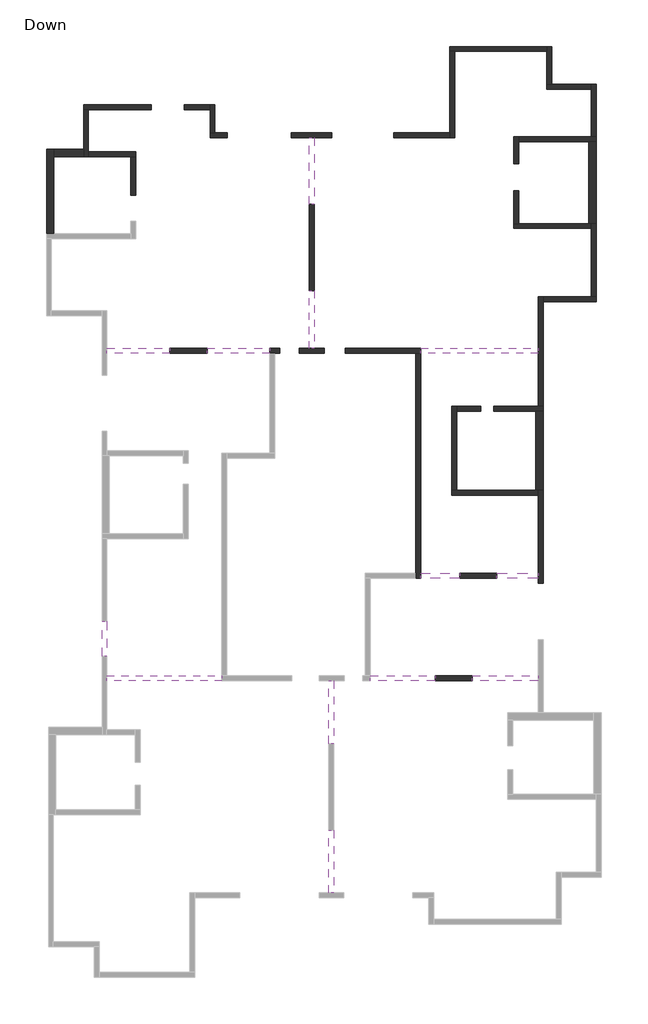
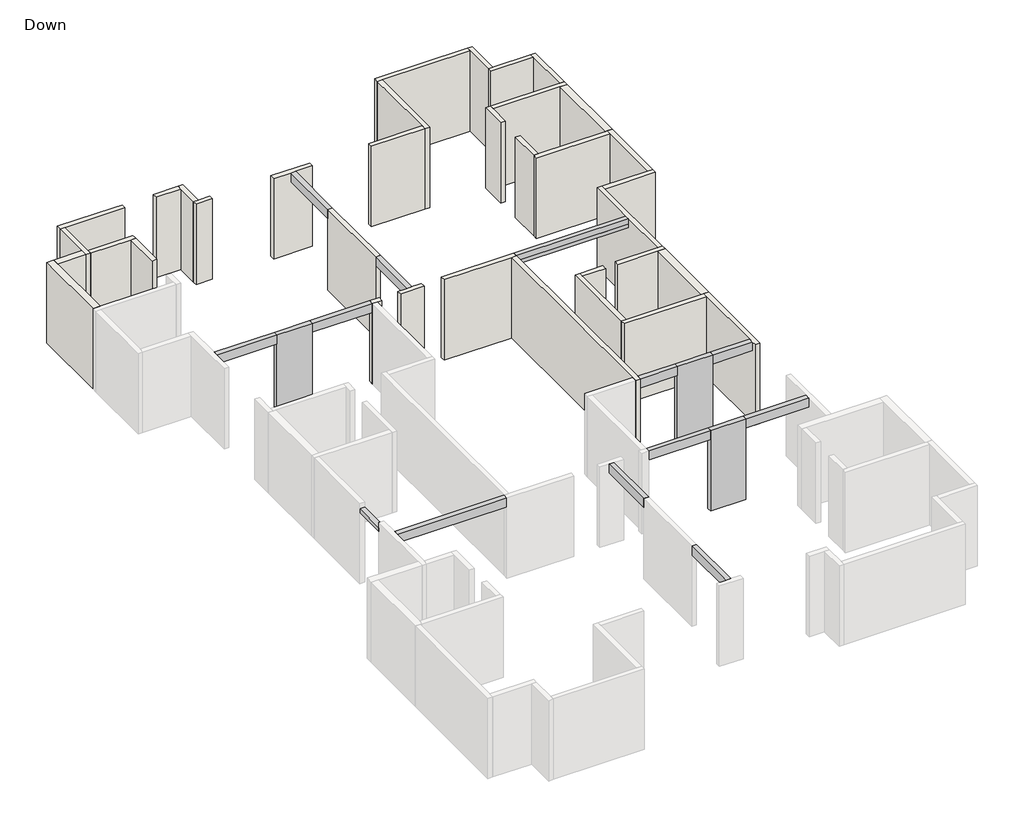
# One storey, part 2 of 2: 35 walls, 13 beams, 3 columns.
"""IFC4 building model written with IfcOpenShell, lengths in millimetres."""

from ifc_helpers import new_model, si_unit, frame, origin, origin_with_axes, place, context, project, spatial, polyline, outline, extrude, faceted_brep, element, save

model = new_model("IFC4")

# Units and contexts
model_context = context("Model", 3, world=origin())
ifc_project = project(units=[si_unit("LENGTHUNIT", "METRE", prefix="MILLI")], contexts=[model_context])

# Site, building, storey
site = spatial("IfcSite", under=ifc_project)
building = spatial("IfcBuilding", under=site)
storey = spatial("IfcBuildingStorey", under=building, Name="Down", Elevation=0.0)

# Beams
placement = place(None, origin())
element("IfcBeam", 1, ObjectType="Concrete Rectengular Beam : 20/40", at=placement, inside=storey, context=model_context, shape_type="Brep", body=[
    faceted_brep([(-3936.3283998, 16023.1258963, 3600.0), (-4136.3283998, 16023.1258963, 3600.0), (-4136.3283998, 16023.1258963, 3200.0), (-3936.3283998, 16023.1258963, 3200.0), (-3936.3283998, 18723.1258963, 3600.0), (-4136.3283998, 18723.1258963, 3600.0), (-4136.3283998, 18723.1258963, 3360.0), (-4136.3283998, 18723.1258963, 3200.0), (-3936.3283998, 18723.1258963, 3200.0), (-3936.3283998, 18723.1258963, 3360.0)], [[[0, 1, 2, 3]], [[1, 0, 4, 5]], [[2, 1, 5, 6, 7]], [[3, 2, 7, 8]], [[0, 3, 8, 9, 4]], [[5, 4, 9, 8, 7, 6]]]),
])
element("IfcBeam", 2, ObjectType="Concrete Rectengular Beam : 20/40", at=placement, inside=storey, context=model_context, shape_type="Brep", body=[
    faceted_brep([(-4136.3283998, 10202.1270927, 3600.0), (-3936.3283998, 10202.1270927, 3600.0), (-3936.3283998, 12523.1258963, 3600.0), (-4136.3283998, 12523.1258963, 3600.0), (-4136.3283998, 10202.1270927, 3200.0), (-4136.3283998, 10202.1270927, 3360.0), (-4136.3283998, 12523.1258963, 3200.0), (-3936.3283998, 10202.1270927, 3200.0), (-3936.3283998, 12523.1258963, 3200.0), (-3936.3283998, 10202.1270927, 3360.0)], [[[0, 1, 2, 3]], [[4, 5, 0, 3, 6]], [[7, 4, 6, 8]], [[1, 9, 7, 8, 2]], [[1, 0, 5, 4, 7, 9]], [[3, 2, 8, 6]]]),
])
element("IfcBeam", 3, ObjectType="Concrete Rectengular Beam : 20/40", at=placement, inside=storey, context=model_context, shape_type="Brep", body=[
    faceted_brep([(-9765.7672932, 10002.1270927, 3600.0), (-9765.7672932, 10202.1270927, 3600.0), (-12310.2559741, 10202.1270927, 3600.0), (-12310.2559741, 10002.1270927, 3600.0), (-9765.7672932, 10002.1270927, 3200.0), (-12310.2559741, 10002.1270927, 3360.0), (-12310.2559741, 10002.1270927, 3200.0), (-9765.7672932, 10202.1270927, 3200.0), (-12310.2559741, 10202.1270927, 3200.0), (-9765.7672932, 10202.1270927, 3360.0), (-12310.2559741, 10202.1270927, 3360.0)], [[[0, 1, 2, 3]], [[4, 0, 3, 5, 6]], [[7, 4, 6, 8]], [[1, 9, 7, 8, 10, 2]], [[1, 0, 4, 7, 9]], [[3, 2, 10, 8, 6, 5]]]),
])
element("IfcBeam", 4, ObjectType="Concrete Rectengular Beam : 20/40", at=placement, inside=storey, context=model_context, shape_type="Brep", body=[
    faceted_brep([(-8265.7672932, 10202.1270927, 3600.0), (-8265.7672932, 10002.1270927, 3600.0), (-5726.5468462, 10002.1270927, 3600.0), (-5726.5468462, 10202.1270927, 3600.0), (-8265.7672932, 10002.1270927, 3200.0), (-5726.5468462, 10002.1270927, 3200.0), (-5726.5468462, 10002.1270927, 3360.0), (-8265.7672932, 10202.1270927, 3200.0), (-5726.5468462, 10202.1270927, 3200.0), (-8265.7672932, 10202.1270927, 3360.0)], [[[0, 1, 2, 3]], [[1, 4, 5, 6, 2]], [[4, 7, 8, 5]], [[7, 9, 0, 3, 8]], [[1, 0, 9, 7, 4]], [[3, 2, 6, 5, 8]]]),
])
element("IfcBeam", 5, ObjectType="Concrete Rectengular Beam : 20/40", at=placement, inside=storey, context=model_context, shape_type="Brep", body=[
    faceted_brep([(365.5355931, 10011.3193389, 3600.0), (5108.6159742, 10011.3193389, 3600.0), (5108.6159742, 10202.1270927, 3600.0), (365.5355931, 10202.1270927, 3600.0), (5108.6159742, 10002.1270927, 3360.0), (365.5355931, 10002.1270927, 3360.0), (365.5355931, 10002.1270927, 3200.0), (5108.6159742, 10002.1270927, 3200.0), (5108.6159742, 10202.1270927, 3200.0), (365.5355931, 10202.1270927, 3200.0), (5108.6159742, 10202.1270927, 3360.0), (5108.6159742, 10011.3193389, 3360.0), (365.5355931, 10011.3193389, 3360.0)], [[[0, 1, 2, 3]], [[4, 5, 6, 7]], [[8, 7, 6, 9]], [[2, 10, 8, 9, 3]], [[11, 12, 5, 4]], [[12, 11, 1, 0]], [[2, 1, 11, 4, 7, 8, 10]], [[0, 3, 9, 6, 5, 12]]]),
])
element("IfcBeam", 6, ObjectType="Concrete Rectengular Beam : 20/40", at=placement, inside=storey, context=model_context, shape_type="Brep", body=[
    faceted_brep([(1935.6692074, 918.1901182, 3600.0), (1935.6692074, 1118.1901182, 3600.0), (365.5355931, 1118.1901182, 3600.0), (365.5355931, 918.1901182, 3600.0), (1935.6692074, 918.1901182, 3200.0), (365.5355931, 918.1901182, 3200.0), (1935.6692074, 1118.1901182, 3200.0), (365.5355931, 1118.1901182, 3200.0), (365.5355931, 1118.1901182, 3360.0)], [[[0, 1, 2, 3]], [[4, 0, 3, 5]], [[6, 4, 5, 7]], [[1, 6, 7, 8, 2]], [[1, 0, 4, 6]], [[3, 2, 8, 7, 5]]]),
])
element("IfcBeam", 7, ObjectType="Concrete Rectengular Beam : 20/40", at=placement, inside=storey, context=model_context, shape_type="Brep", body=[
    faceted_brep([(3435.6692074, 1118.1901182, 3600.0), (3435.6692074, 918.1901182, 3600.0), (5108.6159742, 918.1901182, 3600.0), (5108.6159742, 1118.1901182, 3600.0), (3435.6692074, 918.1901182, 3200.0), (5108.6159742, 918.1901182, 3200.0), (5108.6159742, 918.1901182, 3360.0), (3435.6692074, 1118.1901182, 3200.0), (5108.6159742, 1118.1901182, 3200.0), (5108.6159742, 1118.1901182, 3360.0)], [[[0, 1, 2, 3]], [[1, 4, 5, 6, 2]], [[4, 7, 8, 5]], [[7, 0, 3, 9, 8]], [[1, 0, 7, 4]], [[3, 2, 6, 5, 8, 9]]]),
])
element("IfcBeam", 8, ObjectType="Concrete Rectengular Beam : 20/40", at=placement, inside=storey, context=model_context, shape_type="Brep", body=[
    faceted_brep([(944.6336071, -3227.4112609, 3600.0), (944.6336071, -3027.4112609, 3600.0), (-1668.1246952, -3027.4112609, 3600.0), (-1668.1246952, -3227.4112609, 3600.0), (944.6336071, -3227.4112609, 3200.0), (944.6336071, -3227.4112609, 3360.0), (-1668.1246952, -3227.4112609, 3200.0), (944.6336071, -3027.4112609, 3200.0), (-1668.1246952, -3027.4112609, 3200.0), (-1668.1246952, -3027.4112609, 3360.0)], [[[0, 1, 2, 3]], [[4, 5, 0, 3, 6]], [[7, 4, 6, 8]], [[1, 7, 8, 9, 2]], [[1, 0, 5, 4, 7]], [[3, 2, 9, 8, 6]]]),
])
element("IfcBeam", 9, ObjectType="Concrete Rectengular Beam : 20/40", at=placement, inside=storey, context=model_context, shape_type="Brep", body=[
    faceted_brep([(2444.6336071, -3027.4112609, 3600.0), (2444.6336071, -3227.4112609, 3600.0), (5108.6159742, -3227.4112609, 3600.0), (5108.6159742, -3027.4112609, 3600.0), (2444.6336071, -3227.4112609, 3360.0), (2444.6336071, -3227.4112609, 3200.0), (5108.6159742, -3227.4112609, 3200.0), (5108.6159742, -3227.4112609, 3360.0), (2444.6336071, -3027.4112609, 3200.0), (5108.6159742, -3027.4112609, 3200.0), (5108.6159742, -3027.4112609, 3360.0)], [[[0, 1, 2, 3]], [[1, 4, 5, 6, 7, 2]], [[5, 8, 9, 6]], [[8, 0, 3, 10, 9]], [[1, 0, 8, 5, 4]], [[3, 2, 7, 6, 9, 10]]]),
])
element("IfcBeam", 10, ObjectType="Concrete Rectengular Beam : 20/40", at=placement, inside=storey, context=model_context, shape_type="Brep", body=[
    faceted_brep([(-12310.2559741, -3027.4112609, 3600.0), (-12310.2559741, -3227.4112609, 3600.0), (-7668.2865676, -3227.4112609, 3600.0), (-7668.2865676, -3027.4112609, 3600.0), (-12310.2559741, -3227.4112609, 3360.0), (-12310.2559741, -3227.4112609, 3200.0), (-7668.2865676, -3227.4112609, 3200.0), (-12310.2559741, -3027.4112609, 3200.0), (-7668.2865676, -3027.4112609, 3200.0), (-12310.2559741, -3027.4112609, 3360.0), (-7668.2865676, -3027.4112609, 3360.0)], [[[0, 1, 2, 3]], [[1, 4, 5, 6, 2]], [[5, 7, 8, 6]], [[7, 9, 0, 3, 10, 8]], [[1, 0, 9, 7, 5, 4]], [[3, 2, 6, 8, 10]]]),
])
element("IfcBeam", 11, ObjectType="Concrete Rectengular Beam : 20/40", at=placement, inside=storey, context=model_context, shape_type="Brep", body=[
    faceted_brep([(-3345.8144093, -11796.592326, 3600.0), (-3145.8144093, -11796.592326, 3600.0), (-3145.8144093, -9275.756314, 3600.0), (-3345.8144093, -9275.756314, 3600.0), (-3145.8144093, -11796.592326, 3360.0), (-3145.8144093, -11796.592326, 3200.0), (-3145.8144093, -9275.756314, 3200.0), (-3345.8144093, -11796.592326, 3200.0), (-3345.8144093, -9275.756314, 3200.0), (-3345.8144093, -11796.592326, 3360.0)], [[[0, 1, 2, 3]], [[1, 4, 5, 6, 2]], [[5, 7, 8, 6]], [[7, 9, 0, 3, 8]], [[1, 0, 9, 7, 5, 4]], [[3, 2, 6, 8]]]),
])
element("IfcBeam", 12, ObjectType="Concrete Rectengular Beam : 20/40", at=placement, inside=storey, context=model_context, shape_type="Brep", body=[
    faceted_brep([(-3145.8144093, -3227.4112609, 3600.0), (-3345.8144093, -3227.4112609, 3600.0), (-3345.8144093, -5775.756314, 3600.0), (-3145.8144093, -5775.756314, 3600.0), (-3145.8144093, -3227.4112609, 3200.0), (-3145.8144093, -3227.4112609, 3360.0), (-3145.8144093, -5775.756314, 3200.0), (-3345.8144093, -3227.4112609, 3200.0), (-3345.8144093, -5775.756314, 3200.0), (-3345.8144093, -3227.4112609, 3360.0)], [[[0, 1, 2, 3]], [[4, 5, 0, 3, 6]], [[7, 4, 6, 8]], [[1, 9, 7, 8, 2]], [[1, 0, 5, 4, 7, 9]], [[3, 2, 8, 6]]]),
])
element("IfcBeam", 13, ObjectType="Concrete Rectengular Beam : 20/40", at=placement, inside=storey, context=model_context, shape_type="SweptSolid", body=[
    extrude(outline(polyline([(-12510.2559741, -828.2926655), (-12310.2559741, -828.2926655), (-12310.2559741, -2234.6718166), (-12510.2559741, -2234.6718166), (-12510.2559741, -828.2926655)])), frame((0.0, 0.0, 3200.0), z_axis=(0.0, 0.0, 1.0), x_axis=(1.0, 0.0, 0.0)), (0.0, 0.0, 1.0), 160.0),
])

# Columns
element("IfcColumn", 14, ObjectType="Concrete Rectengular Column : 20/150", at=placement, inside=storey, context=model_context, shape_type="SweptSolid", body=[
    extrude(outline(polyline([(-9765.7672932, 10202.1270927), (-8265.7672932, 10202.1270927), (-8265.7672932, 10002.1270927), (-9765.7672932, 10002.1270927), (-9765.7672932, 10202.1270927)])), origin_with_axes(), (0.0, 0.0, 1.0), 3600.0),
])
element("IfcColumn", 15, ObjectType="Concrete Rectengular Column : 20/150", at=placement, inside=storey, context=model_context, shape_type="SweptSolid", body=[
    extrude(outline(polyline([(1935.6692074, 1118.1901182), (3435.6692074, 1118.1901182), (3435.6692074, 918.1901182), (1935.6692074, 918.1901182), (1935.6692074, 1118.1901182)])), origin_with_axes(), (0.0, 0.0, 1.0), 3600.0),
])
element("IfcColumn", 16, ObjectType="Concrete Rectengular Column : 20/150", at=placement, inside=storey, context=model_context, shape_type="SweptSolid", body=[
    extrude(outline(polyline([(944.6336071, -3027.4112609), (2444.6336071, -3027.4112609), (2444.6336071, -3227.4112609), (944.6336071, -3227.4112609), (944.6336071, -3027.4112609)])), origin_with_axes(), (0.0, 0.0, 1.0), 3600.0),
])

# Walls
element("IfcWall", 17, ObjectType="20", at=placement, inside=storey, context=model_context, shape_type="Brep", body=[
    faceted_brep([(-13057.032521, 17945.140638, 0.0), (-11352.0616697, 17945.140638, 0.0), (-11152.0616697, 17945.140638, 0.0), (-11152.0616697, 17945.140638, 3600.0), (-11352.0616697, 17945.140638, 3600.0), (-13057.032521, 17945.140638, 3600.0), (-13057.032521, 18145.140638, 0.0), (-13057.032521, 18145.140638, 3360.0), (-13057.032521, 18145.140638, 3600.0), (-11152.0616697, 18145.140638, 3600.0), (-11152.0616697, 18145.140638, 3360.0), (-11152.0616697, 18145.140638, 0.0)], [[[0, 1, 2, 3, 4, 5]], [[6, 7, 8, 9, 10, 11]], [[2, 1, 0, 6, 11]], [[5, 4, 3, 9, 8]], [[3, 2, 11, 10, 9]], [[0, 5, 8, 7, 6]]]),
])
element("IfcWall", 18, ObjectType="20", at=placement, inside=storey, context=model_context, shape_type="Brep", body=[
    faceted_brep([(-11352.0616697, 17945.140638, 0.0), (-11352.0616697, 16397.5459604, 0.0), (-11352.0616697, 16397.5459604, 3360.0), (-11352.0616697, 16397.5459604, 3600.0), (-11352.0616697, 17945.140638, 3600.0), (-11352.0616697, 17945.140638, 3360.0), (-11152.0616697, 17945.140638, 0.0), (-11152.0616697, 17945.140638, 3600.0), (-11152.0616697, 16397.5459604, 3600.0), (-11152.0616697, 16397.5459604, 3360.0), (-11152.0616697, 16397.5459604, 0.0)], [[[0, 1, 2, 3, 4, 5]], [[6, 7, 8, 9, 10]], [[1, 0, 6, 10]], [[3, 2, 1, 10, 9, 8]], [[4, 3, 8, 7]], [[0, 5, 4, 7, 6]]]),
])
element("IfcWall", 19, ObjectType="20", at=placement, inside=storey, context=model_context, shape_type="Brep", body=[
    faceted_brep([(5308.6159742, 715.9646069, 0.0), (5308.6159742, 4473.2757833, 0.0), (5308.6159742, 4473.2757833, 3600.0), (5308.6159742, 1278.1901182, 3600.0), (5308.6159742, 715.9646069, 3600.0), (5308.6159742, 715.9646069, 3360.0), (5108.6159742, 715.9646069, 0.0), (5108.6159742, 715.9646069, 3360.0), (5108.6159742, 715.9646069, 3600.0), (5108.6159742, 918.1901182, 3600.0), (5108.6159742, 1118.1901182, 3600.0), (5108.6159742, 4273.2757833, 3600.0), (5108.6159742, 4473.2757833, 3600.0), (5108.6159742, 4473.2757833, 0.0), (5108.6159742, 4273.2757833, 0.0)], [[[0, 1, 2, 3, 4, 5]], [[6, 7, 8, 9, 10, 11, 12, 13, 14]], [[1, 0, 6, 14, 13]], [[4, 3, 2, 12, 11, 10, 9, 8]], [[0, 5, 4, 8, 7, 6]], [[2, 1, 13, 12]]]),
])
element("IfcWall", 20, ObjectType="20", at=placement, inside=storey, context=model_context, shape_type="Brep", body=[
    faceted_brep([(5108.6159742, 4473.2757833, 0.0), (5008.6159742, 4473.2757833, 0.0), (1815.6504069, 4473.2757833, 0.0), (1615.6504069, 4473.2757833, 0.0), (1615.6504069, 4473.2757833, 3600.0), (1815.6504069, 4473.2757833, 3600.0), (5008.6159742, 4473.2757833, 3600.0), (5108.6159742, 4473.2757833, 3600.0), (5108.6159742, 4273.2757833, 0.0), (5108.6159742, 4273.2757833, 3360.0), (5108.6159742, 4273.2757833, 3600.0), (1615.6504069, 4273.2757833, 3600.0), (1615.6504069, 4273.2757833, 3360.0), (1615.6504069, 4273.2757833, 0.0)], [[[0, 1, 2, 3, 4, 5, 6, 7]], [[8, 9, 10, 11, 12, 13]], [[3, 2, 1, 0, 8, 13]], [[7, 6, 5, 4, 11, 10]], [[0, 7, 10, 9, 8]], [[4, 3, 13, 12, 11]]]),
])
element("IfcWall", 21, ObjectType="20", at=placement, inside=storey, context=model_context, shape_type="Brep", body=[
    faceted_brep([(1815.6504069, 4473.2757833, 0.0), (1815.6504069, 7665.1303185, 0.0), (1815.6504069, 7865.1303185, 0.0), (1815.6504069, 7865.1303185, 3600.0), (1815.6504069, 7665.1303185, 3600.0), (1815.6504069, 4473.2757833, 3600.0), (1815.6504069, 4473.2757833, 3360.0), (1615.6504069, 4473.2757833, 0.0), (1615.6504069, 4473.2757833, 3600.0), (1615.6504069, 7865.1303185, 3600.0), (1615.6504069, 7865.1303185, 3360.0), (1615.6504069, 7865.1303185, 0.0)], [[[0, 1, 2, 3, 4, 5, 6]], [[7, 8, 9, 10, 11]], [[2, 1, 0, 7, 11]], [[5, 4, 3, 9, 8]], [[0, 6, 5, 8, 7]], [[3, 2, 11, 10, 9]]]),
])
element("IfcWall", 22, ObjectType="20", at=placement, inside=storey, context=model_context, shape_type="Brep", body=[
    faceted_brep([(3310.841428, 7667.3540488, 0.0), (5008.6159742, 7667.3540488, 0.0), (5308.6159742, 7667.3540488, 0.0), (5308.6159742, 7667.3540488, 3600.0), (5008.6159742, 7667.3540488, 3600.0), (3310.841428, 7667.3540488, 3600.0), (3310.841428, 7667.3540488, 3360.0), (3310.841428, 7867.3540488, 0.0), (3310.841428, 7867.3540488, 3360.0), (3310.841428, 7867.3540488, 3600.0), (5108.6159742, 7867.3540488, 3600.0), (5308.6159742, 7867.3540488, 3600.0), (5308.6159742, 7867.3540488, 0.0), (5108.6159742, 7867.3540488, 0.0)], [[[0, 1, 2, 3, 4, 5, 6]], [[7, 8, 9, 10, 11, 12, 13]], [[2, 1, 0, 7, 13, 12]], [[5, 4, 3, 11, 10, 9]], [[0, 6, 5, 9, 8, 7]], [[3, 2, 12, 11]]]),
])
element("IfcWall", 23, ObjectType="20", at=placement, inside=storey, context=model_context, shape_type="Brep", body=[
    faceted_brep([(5308.6159742, 7867.3540488, 0.0), (5308.6159742, 12088.7143707, 0.0), (5308.6159742, 12288.7143707, 0.0), (5308.6159742, 12288.7143707, 3600.0), (5308.6159742, 12088.7143707, 3600.0), (5308.6159742, 7867.3540488, 3600.0), (5108.6159742, 7867.3540488, 0.0), (5108.6159742, 7867.3540488, 3360.0), (5108.6159742, 7867.3540488, 3600.0), (5108.6159742, 10011.3193389, 3600.0), (5108.6159742, 10202.1270927, 3600.0), (5108.6159742, 12288.7143707, 3600.0), (5108.6159742, 12288.7143707, 3360.0), (5108.6159742, 12288.7143707, 0.0)], [[[0, 1, 2, 3, 4, 5]], [[6, 7, 8, 9, 10, 11, 12, 13]], [[2, 1, 0, 6, 13]], [[5, 4, 3, 11, 10, 9, 8]], [[0, 5, 8, 7, 6]], [[3, 2, 13, 12, 11]]]),
])
element("IfcWall", 24, ObjectType="20", at=placement, inside=storey, context=model_context, shape_type="Brep", body=[
    faceted_brep([(5308.6159742, 12088.7143707, 0.0), (7452.579426, 12088.7143707, 0.0), (7452.579426, 12088.7143707, 3600.0), (5308.6159742, 12088.7143707, 3600.0), (5308.6159742, 12288.7143707, 0.0), (5308.6159742, 12288.7143707, 3600.0), (7252.579426, 12288.7143707, 3600.0), (7452.579426, 12288.7143707, 3600.0), (7452.579426, 12288.7143707, 0.0), (7252.579426, 12288.7143707, 0.0)], [[[0, 1, 2, 3]], [[4, 5, 6, 7, 8, 9]], [[1, 0, 4, 9, 8]], [[3, 2, 7, 6, 5]], [[0, 3, 5, 4]], [[2, 1, 8, 7]]]),
])
element("IfcWall", 25, ObjectType="20", at=placement, inside=storey, context=model_context, shape_type="Brep", body=[
    faceted_brep([(7452.579426, 12288.7143707, 0.0), (7452.579426, 15248.7143707, 0.0), (7452.579426, 15248.7143707, 3600.0), (7452.579426, 12288.7143707, 3600.0), (7252.579426, 12288.7143707, 0.0), (7252.579426, 12288.7143707, 3360.0), (7252.579426, 12288.7143707, 3600.0), (7252.579426, 15048.7143707, 3600.0), (7252.579426, 15248.7143707, 3600.0), (7252.579426, 15248.7143707, 0.0), (7252.579426, 15048.7143707, 0.0)], [[[0, 1, 2, 3]], [[4, 5, 6, 7, 8, 9, 10]], [[1, 0, 4, 10, 9]], [[3, 2, 8, 7, 6]], [[0, 3, 6, 5, 4]], [[2, 1, 9, 8]]]),
])
element("IfcWall", 26, ObjectType="20", at=placement, inside=storey, context=model_context, shape_type="Brep", body=[
    faceted_brep([(7252.579426, 15248.7143707, 0.0), (7152.579426, 15248.7143707, 0.0), (4325.0704423, 15248.7143707, 0.0), (4125.0704423, 15248.7143707, 0.0), (4125.0704423, 15248.7143707, 3600.0), (4325.0704423, 15248.7143707, 3600.0), (7152.579426, 15248.7143707, 3600.0), (7252.579426, 15248.7143707, 3600.0), (7252.579426, 15048.7143707, 0.0), (7252.579426, 15048.7143707, 3360.0), (7252.579426, 15048.7143707, 3600.0), (4125.0704423, 15048.7143707, 3600.0), (4125.0704423, 15048.7143707, 3360.0), (4125.0704423, 15048.7143707, 0.0)], [[[0, 1, 2, 3, 4, 5, 6, 7]], [[8, 9, 10, 11, 12, 13]], [[3, 2, 1, 0, 8, 13]], [[7, 6, 5, 4, 11, 10]], [[0, 7, 10, 9, 8]], [[4, 3, 13, 12, 11]]]),
])
element("IfcWall", 27, ObjectType="20", at=placement, inside=storey, context=model_context, shape_type="Brep", body=[
    faceted_brep([(4325.0704423, 15248.7143707, 0.0), (4325.0704423, 16574.2647824, 0.0), (4325.0704423, 16574.2647824, 3360.0), (4325.0704423, 16574.2647824, 3600.0), (4325.0704423, 15248.7143707, 3600.0), (4325.0704423, 15248.7143707, 3360.0), (4125.0704423, 15248.7143707, 0.0), (4125.0704423, 15248.7143707, 3600.0), (4125.0704423, 16574.2647824, 3600.0), (4125.0704423, 16574.2647824, 3360.0), (4125.0704423, 16574.2647824, 0.0), (4320.0704423, 16574.2647824, 3600.0)], [[[0, 1, 2, 3, 4, 5]], [[6, 7, 8, 9, 10]], [[1, 0, 6, 10]], [[3, 2, 1, 10, 9, 8, 11]], [[4, 3, 11, 8, 7]], [[0, 5, 4, 7, 6]]]),
])
element("IfcWall", 28, ObjectType="20", at=placement, inside=storey, context=model_context, shape_type="Brep", body=[
    faceted_brep([(4325.0704423, 17656.8521012, 0.0), (4325.0704423, 18559.8939047, 0.0), (4325.0704423, 18759.8939047, 0.0), (4325.0704423, 18759.8939047, 3600.0), (4325.0704423, 18559.8939047, 3600.0), (4325.0704423, 17656.8521012, 3600.0), (4325.0704423, 17656.8521012, 3360.0), (4125.0704423, 17656.8521012, 0.0), (4125.0704423, 17656.8521012, 3360.0), (4125.0704423, 17656.8521012, 3600.0), (4125.0704423, 18759.8939047, 3600.0), (4125.0704423, 18759.8939047, 3360.0), (4125.0704423, 18759.8939047, 0.0), (4320.0704423, 17656.8521012, 3600.0)], [[[0, 1, 2, 3, 4, 5, 6]], [[7, 8, 9, 10, 11, 12]], [[2, 1, 0, 7, 12]], [[5, 4, 3, 10, 9, 13]], [[0, 6, 5, 13, 9, 8, 7]], [[3, 2, 12, 11, 10]]]),
])
element("IfcWall", 29, ObjectType="20", at=placement, inside=storey, context=model_context, shape_type="Brep", body=[
    faceted_brep([(4325.0704423, 18559.8939047, 0.0), (7152.579426, 18559.8939047, 0.0), (7452.579426, 18559.8939047, 0.0), (7452.579426, 18559.8939047, 3600.0), (7152.579426, 18559.8939047, 3600.0), (4325.0704423, 18559.8939047, 3600.0), (4325.0704423, 18559.8939047, 3360.0), (4325.0704423, 18759.8939047, 0.0), (4325.0704423, 18759.8939047, 3600.0), (7252.579426, 18759.8939047, 3600.0), (7452.579426, 18759.8939047, 3600.0), (7452.579426, 18759.8939047, 0.0), (7252.579426, 18759.8939047, 0.0)], [[[0, 1, 2, 3, 4, 5, 6]], [[7, 8, 9, 10, 11, 12]], [[2, 1, 0, 7, 12, 11]], [[5, 4, 3, 10, 9, 8]], [[0, 6, 5, 8, 7]], [[3, 2, 11, 10]]]),
])
element("IfcWall", 30, ObjectType="20", at=placement, inside=storey, context=model_context, shape_type="Brep", body=[
    faceted_brep([(7452.579426, 18759.8939047, 0.0), (7452.579426, 20879.8939047, 0.0), (7452.579426, 20879.8939047, 3600.0), (7452.579426, 18759.8939047, 3600.0), (7252.579426, 18759.8939047, 0.0), (7252.579426, 18759.8939047, 3360.0), (7252.579426, 18759.8939047, 3600.0), (7252.579426, 20679.8939047, 3600.0), (7252.579426, 20879.8939047, 3600.0), (7252.579426, 20879.8939047, 0.0), (7252.579426, 20679.8939047, 0.0)], [[[0, 1, 2, 3]], [[4, 5, 6, 7, 8, 9, 10]], [[1, 0, 4, 10, 9]], [[3, 2, 8, 7, 6]], [[0, 3, 6, 5, 4]], [[2, 1, 9, 8]]]),
])
element("IfcWall", 31, ObjectType="20", at=placement, inside=storey, context=model_context, shape_type="Brep", body=[
    faceted_brep([(7252.579426, 20879.8939047, 0.0), (5652.579426, 20879.8939047, 0.0), (5452.579426, 20879.8939047, 0.0), (5452.579426, 20879.8939047, 3600.0), (5652.579426, 20879.8939047, 3600.0), (7252.579426, 20879.8939047, 3600.0), (7252.579426, 20679.8939047, 0.0), (7252.579426, 20679.8939047, 3360.0), (7252.579426, 20679.8939047, 3600.0), (5452.579426, 20679.8939047, 3600.0), (5452.579426, 20679.8939047, 3360.0), (5452.579426, 20679.8939047, 0.0)], [[[0, 1, 2, 3, 4, 5]], [[6, 7, 8, 9, 10, 11]], [[2, 1, 0, 6, 11]], [[5, 4, 3, 9, 8]], [[0, 5, 8, 7, 6]], [[3, 2, 11, 10, 9]]]),
])
element("IfcWall", 32, ObjectType="20", at=placement, inside=storey, context=model_context, shape_type="Brep", body=[
    faceted_brep([(5652.579426, 20879.8939047, 0.0), (5652.579426, 22399.8939047, 0.0), (5652.579426, 22399.8939047, 3600.0), (5652.579426, 20879.8939047, 3600.0), (5452.579426, 20879.8939047, 0.0), (5452.579426, 20879.8939047, 3600.0), (5452.579426, 22199.8939047, 3600.0), (5452.579426, 22399.8939047, 3600.0), (5452.579426, 22399.8939047, 0.0), (5452.579426, 22199.8939047, 0.0)], [[[0, 1, 2, 3]], [[4, 5, 6, 7, 8, 9]], [[1, 0, 4, 9, 8]], [[3, 2, 7, 6, 5]], [[0, 3, 5, 4]], [[2, 1, 8, 7]]]),
])
element("IfcWall", 33, ObjectType="20", at=placement, inside=storey, context=model_context, shape_type="Brep", body=[
    faceted_brep([(5452.579426, 22399.8939047, 0.0), (1532.579426, 22399.8939047, 0.0), (1532.579426, 22399.8939047, 3600.0), (5452.579426, 22399.8939047, 3600.0), (5452.579426, 22199.8939047, 0.0), (5452.579426, 22199.8939047, 3360.0), (5452.579426, 22199.8939047, 3600.0), (1732.579426, 22199.8939047, 3600.0), (1532.579426, 22199.8939047, 3600.0), (1532.579426, 22199.8939047, 0.0), (1732.579426, 22199.8939047, 0.0)], [[[0, 1, 2, 3]], [[4, 5, 6, 7, 8, 9, 10]], [[1, 0, 4, 10, 9]], [[3, 2, 8, 7, 6]], [[0, 3, 6, 5, 4]], [[2, 1, 9, 8]]]),
])
element("IfcWall", 34, ObjectType="20", at=placement, inside=storey, context=model_context, shape_type="Brep", body=[
    faceted_brep([(1532.579426, 22199.8939047, 0.0), (1532.579426, 18923.1258963, 0.0), (1532.579426, 18723.1258963, 0.0), (1532.579426, 18723.1258963, 3600.0), (1532.579426, 18923.1258963, 3600.0), (1532.579426, 21326.7758651, 3600.0), (1532.579426, 22199.8939047, 3600.0), (1732.579426, 22199.8939047, 0.0), (1732.579426, 22199.8939047, 3360.0), (1732.579426, 22199.8939047, 3600.0), (1732.579426, 18723.1258963, 3600.0), (1732.579426, 18723.1258963, 3360.0), (1732.579426, 18723.1258963, 0.0)], [[[0, 1, 2, 3, 4, 5, 6]], [[7, 8, 9, 10, 11, 12]], [[2, 1, 0, 7, 12]], [[6, 5, 4, 3, 10, 9]], [[0, 6, 9, 8, 7]], [[3, 2, 12, 11, 10]]]),
])
element("IfcWall", 35, ObjectType="20", at=placement, inside=storey, context=model_context, shape_type="Brep", body=[
    faceted_brep([(1532.579426, 18923.1258963, 0.0), (-728.3131023, 18923.1258963, 0.0), (-728.3131023, 18923.1258963, 3360.0), (-728.3131023, 18923.1258963, 3600.0), (1532.579426, 18923.1258963, 3600.0), (1532.579426, 18923.1258963, 3360.0), (1532.579426, 18723.1258963, 0.0), (1532.579426, 18723.1258963, 3600.0), (-728.3131023, 18723.1258963, 3600.0), (-728.3131023, 18723.1258963, 3360.0), (-728.3131023, 18723.1258963, 0.0)], [[[0, 1, 2, 3, 4, 5]], [[6, 7, 8, 9, 10]], [[1, 0, 6, 10]], [[3, 2, 1, 10, 9, 8]], [[4, 3, 8, 7]], [[0, 5, 4, 7, 6]]]),
])
element("IfcWall", 36, ObjectType="20", at=placement, inside=storey, context=model_context, shape_type="Brep", body=[
    faceted_brep([(-3228.5427299, 18923.1258963, 0.0), (-4864.7222926, 18923.1258963, 0.0), (-4864.7222926, 18923.1258963, 3360.0), (-4864.7222926, 18923.1258963, 3600.0), (-3228.5427299, 18923.1258963, 3600.0), (-3228.5427299, 18923.1258963, 3360.0), (-3228.5427299, 18723.1258963, 0.0), (-3228.5427299, 18723.1258963, 3360.0), (-3228.5427299, 18723.1258963, 3600.0), (-3936.3283998, 18723.1258963, 3600.0), (-4136.3283998, 18723.1258963, 3600.0), (-4864.7222926, 18723.1258963, 3600.0), (-4864.7222926, 18723.1258963, 3360.0), (-4864.7222926, 18723.1258963, 0.0)], [[[0, 1, 2, 3, 4, 5]], [[6, 7, 8, 9, 10, 11, 12, 13]], [[1, 0, 6, 13]], [[3, 2, 1, 13, 12, 11]], [[4, 3, 11, 10, 9, 8]], [[0, 5, 4, 8, 7, 6]]]),
])
element("IfcWall", 37, ObjectType="20", at=placement, inside=storey, context=model_context, shape_type="Brep", body=[
    faceted_brep([(-7456.8706485, 18923.1258963, 0.0), (-7946.2718834, 18923.1258963, 0.0), (-8146.2718834, 18923.1258963, 0.0), (-8146.2718834, 18923.1258963, 3600.0), (-7946.2718834, 18923.1258963, 3600.0), (-7456.8706485, 18923.1258963, 3600.0), (-7456.8706485, 18923.1258963, 3360.0), (-7456.8706485, 18723.1258963, 0.0), (-7456.8706485, 18723.1258963, 3360.0), (-7456.8706485, 18723.1258963, 3600.0), (-8146.2718834, 18723.1258963, 3600.0), (-8146.2718834, 18723.1258963, 3360.0), (-8146.2718834, 18723.1258963, 0.0)], [[[0, 1, 2, 3, 4, 5, 6]], [[7, 8, 9, 10, 11, 12]], [[2, 1, 0, 7, 12]], [[5, 4, 3, 10, 9]], [[0, 6, 5, 9, 8, 7]], [[3, 2, 12, 11, 10]]]),
])
element("IfcWall", 38, ObjectType="20", at=placement, inside=storey, context=model_context, shape_type="Brep", body=[
    faceted_brep([(-7946.2718834, 18923.1258963, 0.0), (-7946.2718834, 20046.7758651, 0.0), (-7946.2718834, 20046.7758651, 3360.0), (-7946.2718834, 20046.7758651, 3600.0), (-7946.2718834, 18923.1258963, 3600.0), (-7946.2718834, 18923.1258963, 3360.0), (-8146.2718834, 18923.1258963, 0.0), (-8146.2718834, 18923.1258963, 3600.0), (-8146.2718834, 19846.7758651, 3600.0), (-8146.2718834, 20046.7758651, 3600.0), (-8146.2718834, 20046.7758651, 0.0), (-8146.2718834, 19846.7758651, 0.0)], [[[0, 1, 2, 3, 4, 5]], [[6, 7, 8, 9, 10, 11]], [[1, 0, 6, 11, 10]], [[4, 3, 9, 8, 7]], [[0, 5, 4, 7, 6]], [[3, 2, 1, 10, 9]]]),
])
element("IfcWall", 39, ObjectType="20", at=placement, inside=storey, context=model_context, shape_type="Brep", body=[
    faceted_brep([(-8146.2718834, 20046.7758651, 0.0), (-9194.161186, 20046.7758651, 0.0), (-9194.161186, 20046.7758651, 3360.0), (-9194.161186, 20046.7758651, 3600.0), (-8146.2718834, 20046.7758651, 3600.0), (-8146.2718834, 19846.7758651, 0.0), (-8146.2718834, 19846.7758651, 3360.0), (-8146.2718834, 19846.7758651, 3600.0), (-9194.161186, 19846.7758651, 3600.0), (-9194.161186, 19846.7758651, 3360.0), (-9194.161186, 19846.7758651, 0.0)], [[[0, 1, 2, 3, 4]], [[5, 6, 7, 8, 9, 10]], [[1, 0, 5, 10]], [[3, 2, 1, 10, 9, 8]], [[4, 3, 8, 7]], [[0, 4, 7, 6, 5]]]),
])
element("IfcWall", 40, ObjectType="20", at=placement, inside=storey, context=model_context, shape_type="Brep", body=[
    faceted_brep([(-10517.8120165, 20046.7758651, 0.0), (-13257.032521, 20046.7758651, 0.0), (-13257.032521, 20046.7758651, 3600.0), (-10846.2718834, 20046.7758651, 3600.0), (-10517.8120165, 20046.7758651, 3600.0), (-10517.8120165, 20046.7758651, 3360.0), (-10517.8120165, 19846.7758651, 0.0), (-10517.8120165, 19846.7758651, 3360.0), (-10517.8120165, 19846.7758651, 3600.0), (-13057.032521, 19846.7758651, 3600.0), (-13257.032521, 19846.7758651, 3600.0), (-13257.032521, 19846.7758651, 0.0), (-13057.032521, 19846.7758651, 0.0)], [[[0, 1, 2, 3, 4, 5]], [[6, 7, 8, 9, 10, 11, 12]], [[1, 0, 6, 12, 11]], [[4, 3, 2, 10, 9, 8]], [[0, 5, 4, 8, 7, 6]], [[2, 1, 11, 10]]]),
])
element("IfcWall", 41, ObjectType="20", at=placement, inside=storey, context=model_context, shape_type="Brep", body=[
    faceted_brep([(-13257.032521, 19846.7758651, 0.0), (-13257.032521, 18245.140638, 0.0), (-13257.032521, 17945.140638, 0.0), (-13257.032521, 17945.140638, 3600.0), (-13257.032521, 18245.140638, 3600.0), (-13257.032521, 19846.7758651, 3600.0), (-13057.032521, 19846.7758651, 0.0), (-13057.032521, 19846.7758651, 3360.0), (-13057.032521, 19846.7758651, 3600.0), (-13057.032521, 18145.140638, 3600.0), (-13057.032521, 17945.140638, 3600.0), (-13057.032521, 17945.140638, 0.0), (-13057.032521, 18145.140638, 0.0)], [[[0, 1, 2, 3, 4, 5]], [[6, 7, 8, 9, 10, 11, 12]], [[2, 1, 0, 6, 12, 11]], [[5, 4, 3, 10, 9, 8]], [[0, 5, 8, 7, 6]], [[3, 2, 11, 10]]]),
])
element("IfcWall", 42, ObjectType="20", at=placement, inside=storey, context=model_context, shape_type="Brep", body=[
    faceted_brep([(-5726.5468462, 10002.1270927, 0.0), (-5526.5468462, 10002.1270927, 0.0), (-5324.3231159, 10002.1270927, 0.0), (-5324.3231159, 10002.1270927, 3360.0), (-5324.3231159, 10002.1270927, 3600.0), (-5526.5468462, 10002.1270927, 3600.0), (-5726.5468462, 10002.1270927, 3600.0), (-5726.5468462, 10002.1270927, 3200.0), (-5726.5468462, 10202.1270927, 0.0), (-5726.5468462, 10202.1270927, 3200.0), (-5726.5468462, 10202.1270927, 3600.0), (-5324.3231159, 10202.1270927, 3600.0), (-5324.3231159, 10202.1270927, 3360.0), (-5324.3231159, 10202.1270927, 0.0)], [[[0, 1, 2, 3, 4, 5, 6, 7]], [[8, 9, 10, 11, 12, 13]], [[2, 1, 0, 8, 13]], [[4, 3, 2, 13, 12, 11]], [[6, 5, 4, 11, 10]], [[0, 7, 6, 10, 9, 8]]]),
])
element("IfcWall", 43, ObjectType="20", at=placement, inside=storey, context=model_context, shape_type="Brep", body=[
    faceted_brep([(-4533.8091254, 10002.1270927, 0.0), (-3531.8791583, 10002.1270927, 0.0), (-3531.8791583, 10002.1270927, 3600.0), (-4533.8091254, 10002.1270927, 3600.0), (-4533.8091254, 10002.1270927, 3360.0), (-4533.8091254, 10202.1270927, 0.0), (-4533.8091254, 10202.1270927, 3360.0), (-4533.8091254, 10202.1270927, 3600.0), (-4136.3283998, 10202.1270927, 3600.0), (-3936.3283998, 10202.1270927, 3600.0), (-3531.8791583, 10202.1270927, 3600.0), (-3531.8791583, 10202.1270927, 0.0)], [[[0, 1, 2, 3, 4]], [[5, 6, 7, 8, 9, 10, 11]], [[1, 0, 5, 11]], [[2, 1, 11, 10]], [[3, 2, 10, 9, 8, 7]], [[0, 4, 3, 7, 6, 5]]]),
])
element("IfcWall", 44, ObjectType="20", at=placement, inside=storey, context=model_context, shape_type="Brep", body=[
    faceted_brep([(-2686.2135861, 10002.1270927, 0.0), (165.5355931, 10002.1270927, 0.0), (365.5355931, 10002.1270927, 0.0), (365.5355931, 10002.1270927, 3200.0), (365.5355931, 10002.1270927, 3360.0), (365.5355931, 10002.1270927, 3600.0), (165.5355931, 10002.1270927, 3600.0), (-2686.2135861, 10002.1270927, 3600.0), (-2686.2135861, 10002.1270927, 3360.0), (-2686.2135861, 10202.1270927, 0.0), (-2686.2135861, 10202.1270927, 3360.0), (-2686.2135861, 10202.1270927, 3600.0), (365.5355931, 10202.1270927, 3600.0), (365.5355931, 10202.1270927, 3200.0), (365.5355931, 10202.1270927, 0.0), (365.5355931, 10011.3193389, 3600.0)], [[[0, 1, 2, 3, 4, 5, 6, 7, 8]], [[9, 10, 11, 12, 13, 14]], [[2, 1, 0, 9, 14]], [[7, 6, 5, 15, 12, 11]], [[0, 8, 7, 11, 10, 9]], [[5, 4, 3, 2, 14, 13, 12, 15]]]),
])
element("IfcWall", 45, ObjectType="20", at=placement, inside=storey, context=model_context, shape_type="Brep", body=[
    faceted_brep([(165.5355931, 10002.1270927, 0.0), (165.5355931, 1118.1901182, 0.0), (165.5355931, 918.1901182, 0.0), (165.5355931, 918.1901182, 3600.0), (165.5355931, 1118.1901182, 3600.0), (165.5355931, 10002.1270927, 3600.0), (365.5355931, 10002.1270927, 0.0), (365.5355931, 10002.1270927, 3600.0), (365.5355931, 1118.1901182, 3600.0), (365.5355931, 918.1901182, 3600.0), (365.5355931, 918.1901182, 3200.0), (365.5355931, 918.1901182, 0.0)], [[[0, 1, 2, 3, 4, 5]], [[6, 7, 8, 9, 10, 11]], [[2, 1, 0, 6, 11]], [[5, 4, 3, 9, 8, 7]], [[0, 5, 7, 6]], [[3, 2, 11, 10, 9]]]),
])
element("IfcWall", 46, ObjectType="20", at=placement, inside=storey, context=model_context, shape_type="Brep", body=[
    faceted_brep([(2790.841428, 7865.1303185, 0.0), (1815.6504069, 7865.1303185, 0.0), (1815.6504069, 7865.1303185, 3600.0), (2790.841428, 7865.1303185, 3600.0), (2790.841428, 7865.1303185, 3360.0), (2790.841428, 7665.1303185, 0.0), (2790.841428, 7665.1303185, 3360.0), (2790.841428, 7665.1303185, 3600.0), (1815.6504069, 7665.1303185, 3600.0), (1815.6504069, 7665.1303185, 3360.0), (1815.6504069, 7665.1303185, 0.0), (2790.841428, 7667.3540488, 3600.0)], [[[0, 1, 2, 3, 4]], [[5, 6, 7, 8, 9, 10]], [[1, 0, 5, 10]], [[3, 2, 8, 7, 11]], [[0, 4, 3, 11, 7, 6, 5]], [[2, 1, 10, 9, 8]]]),
])
element("IfcWall", 47, ObjectType="20", at=placement, inside=storey, context=model_context, shape_type="Brep", body=[
    faceted_brep([(-4136.3283998, 16023.1258963, 0.0), (-4136.3283998, 12523.1258963, 0.0), (-4136.3283998, 12523.1258963, 3200.0), (-4136.3283998, 12523.1258963, 3600.0), (-4136.3283998, 16023.1258963, 3600.0), (-4136.3283998, 16023.1258963, 3200.0), (-3936.3283998, 16023.1258963, 0.0), (-3936.3283998, 16023.1258963, 3200.0), (-3936.3283998, 16023.1258963, 3600.0), (-3936.3283998, 12523.1258963, 3600.0), (-3936.3283998, 12523.1258963, 3200.0), (-3936.3283998, 12523.1258963, 0.0)], [[[0, 1, 2, 3, 4, 5]], [[6, 7, 8, 9, 10, 11]], [[1, 0, 6, 11]], [[3, 2, 1, 11, 10, 9]], [[4, 3, 9, 8]], [[0, 5, 4, 8, 7, 6]]]),
])
element("IfcWall", 48, ObjectType="30", at=placement, inside=storey, context=model_context, shape_type="Brep", body=[
    faceted_brep([(-14451.9956956, 14832.6787416, 0.0), (-14451.9956956, 17945.140638, 0.0), (-14451.9956956, 18245.140638, 0.0), (-14451.9956956, 18245.140638, 3600.0), (-14451.9956956, 17945.140638, 3600.0), (-14451.9956956, 14832.6787416, 3600.0), (-14451.9956956, 14832.6787416, 3360.0), (-14751.9956956, 14832.6787416, 0.0), (-14751.9956956, 14832.6787416, 3600.0), (-14751.9956956, 18245.140638, 3600.0), (-14751.9956956, 18245.140638, 0.0)], [[[0, 1, 2, 3, 4, 5, 6]], [[7, 8, 9, 10]], [[2, 1, 0, 7, 10]], [[5, 4, 3, 9, 8]], [[3, 2, 10, 9]], [[0, 6, 5, 8, 7]]]),
])
element("IfcWall", 49, ObjectType="30", at=placement, inside=storey, context=model_context, shape_type="Brep", body=[
    faceted_brep([(-14451.9956956, 17945.140638, 0.0), (-13257.032521, 17945.140638, 0.0), (-13257.032521, 17945.140638, 3600.0), (-14451.9956956, 17945.140638, 3600.0), (-14451.9956956, 17945.140638, 3360.0), (-14451.9956956, 18245.140638, 0.0), (-14451.9956956, 18245.140638, 3600.0), (-13257.032521, 18245.140638, 3600.0), (-13257.032521, 18245.140638, 0.0)], [[[0, 1, 2, 3, 4]], [[5, 6, 7, 8]], [[1, 0, 5, 8]], [[3, 2, 7, 6]], [[0, 4, 3, 6, 5]], [[2, 1, 8, 7]]]),
])
element("IfcWall", 50, ObjectType="30", at=placement, inside=storey, context=model_context, shape_type="Brep", body=[
    faceted_brep([(5008.6159742, 7667.3540488, 0.0), (5008.6159742, 4473.2757833, 0.0), (5008.6159742, 4473.2757833, 3360.0), (5008.6159742, 4473.2757833, 3600.0), (5008.6159742, 7667.3540488, 3600.0), (5008.6159742, 7667.3540488, 3360.0), (5308.6159742, 7667.3540488, 0.0), (5308.6159742, 7667.3540488, 3600.0), (5308.6159742, 4473.2757833, 3600.0), (5308.6159742, 4473.2757833, 0.0), (5108.6159742, 4473.2757833, 0.0), (5108.6159742, 4473.2757833, 3600.0)], [[[0, 1, 2, 3, 4, 5]], [[6, 7, 8, 9]], [[1, 0, 6, 9, 10]], [[4, 3, 11, 8, 7]], [[3, 2, 1, 10, 9, 8, 11]], [[0, 5, 4, 7, 6]]]),
])
element("IfcWall", 51, ObjectType="30", at=placement, inside=storey, context=model_context, shape_type="Brep", body=[
    faceted_brep([(7152.579426, 18559.8939047, 0.0), (7152.579426, 15248.7143707, 0.0), (7152.579426, 15248.7143707, 3360.0), (7152.579426, 15248.7143707, 3600.0), (7152.579426, 18559.8939047, 3600.0), (7152.579426, 18559.8939047, 3360.0), (7452.579426, 18559.8939047, 0.0), (7452.579426, 18559.8939047, 3600.0), (7452.579426, 15248.7143707, 3600.0), (7452.579426, 15248.7143707, 0.0), (7252.579426, 15248.7143707, 0.0), (7252.579426, 15248.7143707, 3600.0)], [[[0, 1, 2, 3, 4, 5]], [[6, 7, 8, 9]], [[1, 0, 6, 9, 10]], [[4, 3, 11, 8, 7]], [[0, 5, 4, 7, 6]], [[3, 2, 1, 10, 9, 8, 11]]]),
])

save(model, "model.ifc")

# Revit data of these elements
# Type "Concrete Rectengular Beam : 20/40"
#   Keynote = "09000"
#   Length [instance default] = 152.4 cm
#   b = 20 cm
#   h = 40 cm
#   Structural Material [instance default] = Concrete
#   Assembly Code = ""
# Type "Concrete Rectengular Column : 20/150"
#   b = 20 cm
#   h = 150 cm
#   Structural Material [instance default] = Concrete
# Type "20"
#   Layers, outside or top first: 20 cm "Concrete" (function 1)
# Type "30"
#   Layers, outside or top first: 30 cm "Concrete" (function 1)
# Element 1 (IfcBeam, "Concrete Rectengular Beam : 20/40")
#   Comments = ""
#   Mark = "B1"
#   SOFiSTiK_AMG_Comments = ""
#   SOFiSTiK_AMG_Scheduled = yes
#   SOFiSTiK_AMG_Adjusted = yes
#   Structural Material = Concrete
#   Phase Created = New Construction
#   Materials on its faces: "Concrete"
# Element 2 (IfcBeam, "Concrete Rectengular Beam : 20/40")
#   Comments = ""
#   Mark = "B2"
#   SOFiSTiK_AMG_Comments = ""
#   SOFiSTiK_AMG_Scheduled = yes
#   SOFiSTiK_AMG_Adjusted = yes
#   Structural Material = Concrete
#   Phase Created = New Construction
#   Materials on its faces: "Concrete"
# Element 3 (IfcBeam, "Concrete Rectengular Beam : 20/40")
#   Comments = ""
#   Mark = "B3"
#   SOFiSTiK_AMG_Comments = ""
#   SOFiSTiK_AMG_Scheduled = yes
#   SOFiSTiK_AMG_Adjusted = yes
#   Structural Material = Concrete
#   Phase Created = New Construction
#   Materials on its faces: "Concrete"
# Element 4 (IfcBeam, "Concrete Rectengular Beam : 20/40")
#   Comments = ""
#   Mark = "B4"
#   SOFiSTiK_AMG_Comments = ""
#   SOFiSTiK_AMG_Scheduled = yes
#   SOFiSTiK_AMG_Adjusted = yes
#   Structural Material = Concrete
#   Phase Created = New Construction
#   Materials on its faces: "Concrete"
# Element 5 (IfcBeam, "Concrete Rectengular Beam : 20/40")
#   Comments = ""
#   Mark = "B5"
#   SOFiSTiK_AMG_Comments = ""
#   SOFiSTiK_AMG_Scheduled = yes
#   SOFiSTiK_AMG_Adjusted = yes
#   Structural Material = Concrete
#   Phase Created = New Construction
#   Materials on its faces: "Concrete"
# Element 6 (IfcBeam, "Concrete Rectengular Beam : 20/40")
#   Comments = ""
#   Mark = "B6"
#   SOFiSTiK_AMG_Comments = ""
#   SOFiSTiK_AMG_Scheduled = yes
#   SOFiSTiK_AMG_Adjusted = yes
#   Structural Material = Concrete
#   Phase Created = New Construction
#   Materials on its faces: "Concrete"
# Element 7 (IfcBeam, "Concrete Rectengular Beam : 20/40")
#   Comments = ""
#   Mark = "B7"
#   SOFiSTiK_AMG_Comments = ""
#   SOFiSTiK_AMG_Scheduled = yes
#   SOFiSTiK_AMG_Adjusted = yes
#   Structural Material = Concrete
#   Phase Created = New Construction
#   Materials on its faces: "Concrete"
# Element 8 (IfcBeam, "Concrete Rectengular Beam : 20/40")
#   Comments = ""
#   Mark = "B8"
#   SOFiSTiK_AMG_Comments = ""
#   SOFiSTiK_AMG_Scheduled = yes
#   SOFiSTiK_AMG_Adjusted = yes
#   Structural Material = Concrete
#   Phase Created = New Construction
#   Materials on its faces: "Concrete"
# Element 9 (IfcBeam, "Concrete Rectengular Beam : 20/40")
#   Comments = ""
#   Mark = "B9"
#   SOFiSTiK_AMG_Comments = ""
#   SOFiSTiK_AMG_Scheduled = yes
#   SOFiSTiK_AMG_Adjusted = yes
#   Structural Material = Concrete
#   Phase Created = New Construction
#   Materials on its faces: "Concrete"
# Element 10 (IfcBeam, "Concrete Rectengular Beam : 20/40")
#   Comments = ""
#   Mark = "B10"
#   SOFiSTiK_AMG_Comments = ""
#   SOFiSTiK_AMG_Scheduled = yes
#   SOFiSTiK_AMG_Adjusted = yes
#   Structural Material = Concrete
#   Phase Created = New Construction
#   Materials on its faces: "Concrete"
# Element 11 (IfcBeam, "Concrete Rectengular Beam : 20/40")
#   Comments = ""
#   Mark = "B11"
#   SOFiSTiK_AMG_Comments = ""
#   SOFiSTiK_AMG_Scheduled = yes
#   SOFiSTiK_AMG_Adjusted = yes
#   Structural Material = Concrete
#   Phase Created = New Construction
#   Materials on its faces: "Concrete"
# Element 12 (IfcBeam, "Concrete Rectengular Beam : 20/40")
#   Comments = ""
#   Mark = "B12"
#   SOFiSTiK_AMG_Comments = ""
#   SOFiSTiK_AMG_Scheduled = yes
#   SOFiSTiK_AMG_Adjusted = yes
#   Structural Material = Concrete
#   Phase Created = New Construction
#   Materials on its faces: "Concrete"
# Element 13 (IfcBeam, "Concrete Rectengular Beam : 20/40")
#   Comments = ""
#   Mark = "B13"
#   SOFiSTiK_AMG_Comments = ""
#   SOFiSTiK_AMG_Scheduled = yes
#   SOFiSTiK_AMG_Adjusted = yes
#   Structural Material = Concrete
#   Phase Created = New Construction
#   Materials on its faces: "Concrete"
# Element 14 (IfcColumn, "Concrete Rectengular Column : 20/150")
#   Comments = ""
#   Mark = "C1"
#   SOFiSTiK_AMG_Comments = ""
#   SOFiSTiK_AMG_Scheduled = yes
#   SOFiSTiK_AMG_Adjusted = yes
#   Structural Material = Concrete
#   Phase Created = New Construction
#   Materials on its faces: "Concrete"
# Element 15 (IfcColumn, "Concrete Rectengular Column : 20/150")
#   Comments = ""
#   Mark = "C2"
#   SOFiSTiK_AMG_Comments = ""
#   SOFiSTiK_AMG_Scheduled = yes
#   SOFiSTiK_AMG_Adjusted = yes
#   Structural Material = Concrete
#   Phase Created = New Construction
#   Materials on its faces: "Concrete"
# Element 16 (IfcColumn, "Concrete Rectengular Column : 20/150")
#   Comments = ""
#   Mark = "C3"
#   SOFiSTiK_AMG_Comments = ""
#   SOFiSTiK_AMG_Scheduled = yes
#   SOFiSTiK_AMG_Adjusted = yes
#   Structural Material = Concrete
#   Phase Created = New Construction
#   Materials on its faces: "Concrete"
# Element 17 (IfcWall, "20")
#   Comments = ""
#   Mark = "W10"
#   SOFiSTiK_EdgeZones = "W11"
#   SOFiSTiK_AMG_Comments = ""
#   Top Offset = 0 cm
#   Base Offset = 0 cm
#   wall height = 360 cm
#   SOFiSTiK_AMG_Scheduled = yes
#   SOFiSTiK_AMG_Adjusted = yes
#   Phase Created = New Construction
#   Base Constraint = Down
#   Top Constraint = Typical Floor
#   Materials on its faces: "Concrete"
# Element 18 (IfcWall, "20")
#   Comments = ""
#   Mark = "W11"
#   SOFiSTiK_EdgeZones = "W12"
#   SOFiSTiK_AMG_Comments = ""
#   Top Offset = 0 cm
#   Base Offset = 0 cm
#   wall height = 360 cm
#   SOFiSTiK_AMG_Scheduled = yes
#   SOFiSTiK_AMG_Adjusted = yes
#   Phase Created = New Construction
#   Base Constraint = Down
#   Top Constraint = Typical Floor
#   Materials on its faces: "Concrete"
# Element 19 (IfcWall, "20")
#   Comments = ""
#   Mark = "W45"
#   SOFiSTiK_EdgeZones = "W46"
#   SOFiSTiK_AMG_Comments = ""
#   Top Offset = 0 cm
#   Base Offset = 0 cm
#   wall height = 360 cm
#   SOFiSTiK_AMG_Scheduled = yes
#   SOFiSTiK_AMG_Adjusted = yes
#   Phase Created = New Construction
#   Base Constraint = Down
#   Top Constraint = Typical Floor
#   Materials on its faces: "Concrete"
# Element 20 (IfcWall, "20")
#   Comments = ""
#   Mark = "W46"
#   SOFiSTiK_EdgeZones = "W47"
#   SOFiSTiK_AMG_Comments = ""
#   Top Offset = 0 cm
#   Base Offset = 0 cm
#   wall height = 360 cm
#   SOFiSTiK_AMG_Scheduled = yes
#   SOFiSTiK_AMG_Adjusted = yes
#   Phase Created = New Construction
#   Base Constraint = Down
#   Top Constraint = Typical Floor
#   Materials on its faces: "Concrete"
# Element 21 (IfcWall, "20")
#   Comments = ""
#   Mark = "W47"
#   SOFiSTiK_EdgeZones = "W48"
#   SOFiSTiK_AMG_Comments = ""
#   Top Offset = 0 cm
#   Base Offset = 0 cm
#   wall height = 360 cm
#   SOFiSTiK_AMG_Scheduled = yes
#   SOFiSTiK_AMG_Adjusted = yes
#   Phase Created = New Construction
#   Base Constraint = Down
#   Top Constraint = Typical Floor
#   Materials on its faces: "Concrete"
# Element 22 (IfcWall, "20")
#   Comments = ""
#   Mark = "W48"
#   SOFiSTiK_EdgeZones = "W49"
#   SOFiSTiK_AMG_Comments = ""
#   Top Offset = 0 cm
#   Base Offset = 0 cm
#   wall height = 360 cm
#   SOFiSTiK_AMG_Scheduled = yes
#   SOFiSTiK_AMG_Adjusted = yes
#   Phase Created = New Construction
#   Base Constraint = Down
#   Top Constraint = Typical Floor
#   Materials on its faces: "Concrete"
# Element 23 (IfcWall, "20")
#   Comments = ""
#   Mark = "W49"
#   SOFiSTiK_EdgeZones = "W50"
#   SOFiSTiK_AMG_Comments = ""
#   Top Offset = 0 cm
#   Base Offset = 0 cm
#   wall height = 360 cm
#   SOFiSTiK_AMG_Scheduled = yes
#   SOFiSTiK_AMG_Adjusted = yes
#   Phase Created = New Construction
#   Base Constraint = Down
#   Top Constraint = Typical Floor
#   Materials on its faces: "Concrete"
# Element 24 (IfcWall, "20")
#   Comments = ""
#   Mark = "W50"
#   SOFiSTiK_EdgeZones = "W51"
#   SOFiSTiK_AMG_Comments = ""
#   Top Offset = 0 cm
#   Base Offset = 0 cm
#   wall height = 360 cm
#   SOFiSTiK_AMG_Scheduled = yes
#   SOFiSTiK_AMG_Adjusted = yes
#   Phase Created = New Construction
#   Base Constraint = Down
#   Top Constraint = Typical Floor
#   Materials on its faces: "Concrete"
# Element 25 (IfcWall, "20")
#   Comments = ""
#   Mark = "W51"
#   SOFiSTiK_EdgeZones = "W52"
#   SOFiSTiK_AMG_Comments = ""
#   Top Offset = 0 cm
#   Base Offset = 0 cm
#   wall height = 360 cm
#   SOFiSTiK_AMG_Scheduled = yes
#   SOFiSTiK_AMG_Adjusted = yes
#   Phase Created = New Construction
#   Base Constraint = Down
#   Top Constraint = Typical Floor
#   Materials on its faces: "Concrete"
# Element 26 (IfcWall, "20")
#   Comments = ""
#   Mark = "W52"
#   SOFiSTiK_EdgeZones = "W53"
#   SOFiSTiK_AMG_Comments = ""
#   Top Offset = 0 cm
#   Base Offset = 0 cm
#   wall height = 360 cm
#   SOFiSTiK_AMG_Scheduled = yes
#   SOFiSTiK_AMG_Adjusted = yes
#   Phase Created = New Construction
#   Base Constraint = Down
#   Top Constraint = Typical Floor
#   Materials on its faces: "Concrete"
# Element 27 (IfcWall, "20")
#   Comments = ""
#   Mark = "W53"
#   SOFiSTiK_EdgeZones = "W54"
#   SOFiSTiK_AMG_Comments = ""
#   Top Offset = 0 cm
#   Base Offset = 0 cm
#   wall height = 360 cm
#   SOFiSTiK_AMG_Scheduled = yes
#   SOFiSTiK_AMG_Adjusted = yes
#   Phase Created = New Construction
#   Base Constraint = Down
#   Top Constraint = Typical Floor
#   Materials on its faces: "Concrete"
# Element 28 (IfcWall, "20")
#   Comments = ""
#   Mark = "W54"
#   SOFiSTiK_EdgeZones = "W55"
#   SOFiSTiK_AMG_Comments = ""
#   Top Offset = 0 cm
#   Base Offset = 0 cm
#   wall height = 360 cm
#   SOFiSTiK_AMG_Scheduled = yes
#   SOFiSTiK_AMG_Adjusted = yes
#   Phase Created = New Construction
#   Base Constraint = Down
#   Top Constraint = Typical Floor
#   Materials on its faces: "Concrete"
# Element 29 (IfcWall, "20")
#   Comments = ""
#   Mark = "W55"
#   SOFiSTiK_EdgeZones = "W56"
#   SOFiSTiK_AMG_Comments = ""
#   Top Offset = 0 cm
#   Base Offset = 0 cm
#   wall height = 360 cm
#   SOFiSTiK_AMG_Scheduled = yes
#   SOFiSTiK_AMG_Adjusted = yes
#   Phase Created = New Construction
#   Base Constraint = Down
#   Top Constraint = Typical Floor
#   Materials on its faces: "Concrete"
# Element 30 (IfcWall, "20")
#   Comments = ""
#   Mark = "W56"
#   SOFiSTiK_EdgeZones = "W57"
#   SOFiSTiK_AMG_Comments = ""
#   Top Offset = 0 cm
#   Base Offset = 0 cm
#   wall height = 360 cm
#   SOFiSTiK_AMG_Scheduled = yes
#   SOFiSTiK_AMG_Adjusted = yes
#   Phase Created = New Construction
#   Base Constraint = Down
#   Top Constraint = Typical Floor
#   Materials on its faces: "Concrete"
# Element 31 (IfcWall, "20")
#   Comments = ""
#   Mark = "W57"
#   SOFiSTiK_EdgeZones = "W58"
#   SOFiSTiK_AMG_Comments = ""
#   Top Offset = 0 cm
#   Base Offset = 0 cm
#   wall height = 360 cm
#   SOFiSTiK_AMG_Scheduled = yes
#   SOFiSTiK_AMG_Adjusted = yes
#   Phase Created = New Construction
#   Base Constraint = Down
#   Top Constraint = Typical Floor
#   Materials on its faces: "Concrete"
# Element 32 (IfcWall, "20")
#   Comments = ""
#   Mark = "W58"
#   SOFiSTiK_EdgeZones = "W59"
#   SOFiSTiK_AMG_Comments = ""
#   Top Offset = 0 cm
#   Base Offset = 0 cm
#   wall height = 360 cm
#   SOFiSTiK_AMG_Scheduled = yes
#   SOFiSTiK_AMG_Adjusted = yes
#   Phase Created = New Construction
#   Base Constraint = Down
#   Top Constraint = Typical Floor
#   Materials on its faces: "Concrete"
# Element 33 (IfcWall, "20")
#   Comments = ""
#   Mark = "W59"
#   SOFiSTiK_EdgeZones = "W60"
#   SOFiSTiK_AMG_Comments = ""
#   Top Offset = 0 cm
#   Base Offset = 0 cm
#   wall height = 360 cm
#   SOFiSTiK_AMG_Scheduled = yes
#   SOFiSTiK_AMG_Adjusted = yes
#   Phase Created = New Construction
#   Base Constraint = Down
#   Top Constraint = Typical Floor
#   Materials on its faces: "Concrete"
# Element 34 (IfcWall, "20")
#   Comments = ""
#   Mark = "W60"
#   SOFiSTiK_EdgeZones = "W61"
#   SOFiSTiK_AMG_Comments = ""
#   Top Offset = 0 cm
#   Base Offset = 0 cm
#   wall height = 360 cm
#   SOFiSTiK_AMG_Scheduled = yes
#   SOFiSTiK_AMG_Adjusted = yes
#   Phase Created = New Construction
#   Base Constraint = Down
#   Top Constraint = Typical Floor
#   Materials on its faces: "Concrete"
# Element 35 (IfcWall, "20")
#   Comments = ""
#   Mark = "W61"
#   SOFiSTiK_EdgeZones = "W62"
#   SOFiSTiK_AMG_Comments = ""
#   Top Offset = 0 cm
#   Base Offset = 0 cm
#   wall height = 360 cm
#   SOFiSTiK_AMG_Scheduled = yes
#   SOFiSTiK_AMG_Adjusted = yes
#   Phase Created = New Construction
#   Base Constraint = Down
#   Top Constraint = Typical Floor
#   Materials on its faces: "Concrete"
# Element 36 (IfcWall, "20")
#   Comments = ""
#   Mark = "W62"
#   SOFiSTiK_EdgeZones = "W63"
#   SOFiSTiK_AMG_Comments = ""
#   Top Offset = 0 cm
#   Base Offset = 0 cm
#   wall height = 360 cm
#   SOFiSTiK_AMG_Scheduled = yes
#   SOFiSTiK_AMG_Adjusted = yes
#   Phase Created = New Construction
#   Base Constraint = Down
#   Top Constraint = Typical Floor
#   Materials on its faces: "Concrete"
# Element 37 (IfcWall, "20")
#   Comments = ""
#   Mark = "W63"
#   SOFiSTiK_EdgeZones = "W64"
#   SOFiSTiK_AMG_Comments = ""
#   Top Offset = 0 cm
#   Base Offset = 0 cm
#   wall height = 360 cm
#   SOFiSTiK_AMG_Scheduled = yes
#   SOFiSTiK_AMG_Adjusted = yes
#   Phase Created = New Construction
#   Base Constraint = Down
#   Top Constraint = Typical Floor
#   Materials on its faces: "Concrete"
# Element 38 (IfcWall, "20")
#   Comments = ""
#   Mark = "W64"
#   SOFiSTiK_EdgeZones = "W65"
#   SOFiSTiK_AMG_Comments = ""
#   Top Offset = 0 cm
#   Base Offset = 0 cm
#   wall height = 360 cm
#   SOFiSTiK_AMG_Scheduled = yes
#   SOFiSTiK_AMG_Adjusted = yes
#   Phase Created = New Construction
#   Base Constraint = Down
#   Top Constraint = Typical Floor
#   Materials on its faces: "Concrete"
# Element 39 (IfcWall, "20")
#   Comments = ""
#   Mark = "W65"
#   SOFiSTiK_EdgeZones = "W66"
#   SOFiSTiK_AMG_Comments = ""
